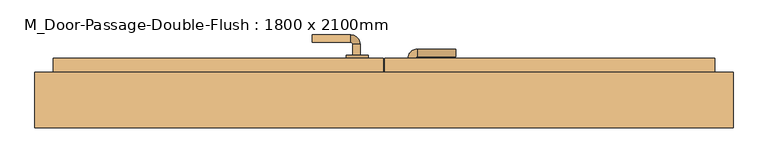
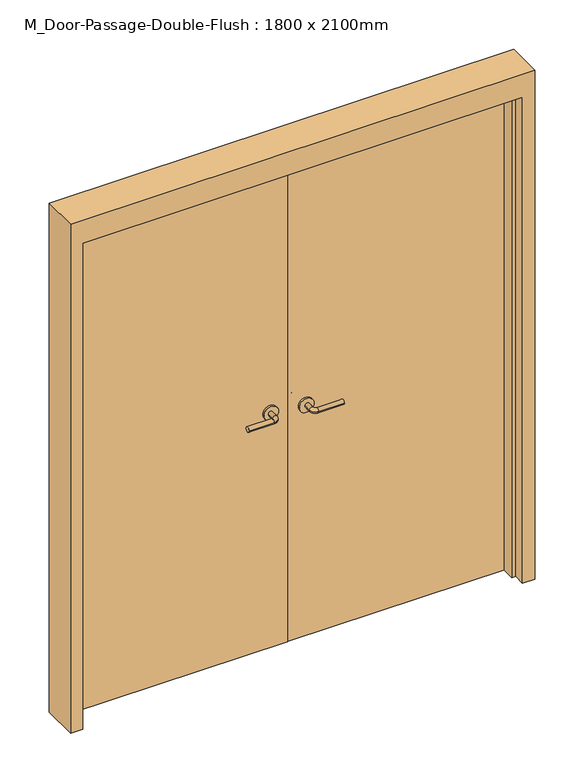
"""IFC4 building model written with IfcOpenShell, lengths in millimetres: door geometry, M_Door-Passage-Double-Flush : 1800 x 2100mm."""

from ifc_helpers import new_model, si_unit, point, frame, frame_2d, origin, origin_with_axes, place, context, project, spatial, polyline, circle_curve, ellipse_curve, trimmed, segment, composite_curve, outline, extrude, faceted_brep, source, transform, mapped, element, save
from ifc_brep_helpers import plane_surface, cylinder_surface, revolved_surface, advanced_brep


def m_door_passage_double_flush_1800_x_2100mm_c8e1a3e4(model_context):
    return source(origin(), model_context, "Body", "SolidModel", [
        advanced_brep(
        [(-65.009375, -9.15, 1016.0), (-85.009375, -9.15, 1016.0), (-65.009375, -39.15, 1016.0), (-85.009375, -39.15, 1016.0), (-90.009375, -44.15, 1016.0), (-90.009375, -64.15, 1016.0), (-195.009375, -64.15, 1016.0), (-195.009375, -44.15, 1016.0)],
        [
            (0, 1, circle_curve(frame((-75.009375, -9.15, 1016.0), z_axis=(0.0, 1.0, 0.0), x_axis=(-1.0, 0.0, 0.0)), 10.0)),
            (1, 0, circle_curve(frame((-75.009375, -9.15, 1016.0), z_axis=(0.0, 1.0, 0.0), x_axis=(-1.0, 0.0, 0.0)), 10.0)),
            (0, 2),
            (2, 3, circle_curve(frame((-75.009375, -39.15, 1016.0), z_axis=(0.0, 1.0, 0.0), x_axis=(-1.0, 0.0, 0.0)), 10.0)),
            (3, 1),
            (3, 2, circle_curve(frame((-75.009375, -39.15, 1016.0), z_axis=(0.0, 1.0, 0.0), x_axis=(-1.0, 0.0, 0.0)), 10.0)),
            (4, 3, circle_curve(frame((-90.009375, -39.15, 1016.0), z_axis=(0.0, 0.0, 1.0), x_axis=(1.0, 0.0, 0.0)), 5.0)),
            (2, 5, circle_curve(frame((-90.009375, -39.15, 1016.0), z_axis=(0.0, 0.0, -1.0), x_axis=(1.0, 0.0, 0.0)), 25.0)),
            (5, 4, circle_curve(frame((-90.009375, -54.15, 1016.0), z_axis=(1.0, 0.0, 0.0), x_axis=(0.0, 1.0, 0.0)), 10.0)),
            (4, 5, circle_curve(frame((-90.009375, -54.15, 1016.0), z_axis=(1.0, 0.0, 0.0), x_axis=(0.0, 1.0, 0.0)), 10.0)),
            (6, 7, circle_curve(frame((-195.009375, -54.15, 1016.0), z_axis=(-1.0, 0.0, 0.0), x_axis=(0.0, 1.0, 0.0)), 10.0)),
            (7, 6, circle_curve(frame((-195.009375, -54.15, 1016.0), z_axis=(-1.0, 0.0, 0.0), x_axis=(0.0, 1.0, 0.0)), 10.0)),
            (5, 6),
            (7, 4),
        ],
        [
            plane_surface(frame((-75.009375, -9.15, 1016.0), z_axis=(0.0, 1.0, 0.0), x_axis=(0.0, 0.0, 1.0))),
            cylinder_surface(frame((-75.009375, -9.15, 1016.0), z_axis=(0.0, 1.0, 0.0), x_axis=(-1.0, 0.0, 0.0)), 10.0),
            revolved_surface(trimmed(ellipse_curve(frame((-75.009375, -39.15, 1016.0), z_axis=(0.0, 1.0, 0.0), x_axis=(-1.0, 0.0, 0.0)), 10.0, 10.0), [point((-65.009375, -39.15, 1016.0))], [point((-85.009375, -39.15, 1016.0))], True, "CARTESIAN"), (-90.009375, -39.15, 1016.0), (0.0, 0.0, -1.0)),
            revolved_surface(trimmed(ellipse_curve(frame((-75.009375, -39.15, 1016.0), z_axis=(0.0, 1.0, 0.0), x_axis=(-1.0, 0.0, 0.0)), 10.0, 10.0), [point((-85.009375, -39.15, 1016.0))], [point((-65.009375, -39.15, 1016.0))], True, "CARTESIAN"), (-90.009375, -39.15, 1016.0), (0.0, 0.0, -1.0)),
            plane_surface(frame((-195.009375, -54.15, 1016.0), z_axis=(-1.0, 0.0, 0.0), x_axis=(0.0, 0.0, 1.0))),
            cylinder_surface(frame((-90.009375, -54.15, 1016.0), z_axis=(1.0, 0.0, 0.0), x_axis=(0.0, 1.0, 0.0)), 10.0),
        ],
        [
            (0, [[1, 2]]),
            (1, [[-1, 3, 4, 5]]),
            (1, [[-2, -5, 6, -3]]),
            (2, [[7, -4, 8, 9]]),
            (3, [[-8, -6, -7, 10]]),
            (4, [[11, 12]]),
            (5, [[-9, 13, -12, 14]]),
            (5, [[-10, -14, -11, -13]]),
        ],
    ),
        extrude(outline(composite_curve([segment(trimmed(circle_curve(frame_2d((1016.0, -72.509375)), 30.0), [point((1016.0, -42.509375))], [point((1016.0, -102.509375))], False, "CARTESIAN"), True, "CONTINUOUS"), segment(trimmed(circle_curve(frame_2d((1016.0, -72.509375)), 30.0), [point((1016.0, -102.509375))], [point((1016.0, -42.509375))], False, "CARTESIAN"), True, "CONTINUOUS")], self_intersect=False)), frame((0.0, -9.15, 0.0), z_axis=(0.0, 1.0, 0.0), x_axis=(0.0, 0.0, 1.0)), (0.0, 0.0, 1.0), 8.0),
        advanced_brep(
        [(-65.009375, 90.95, 1000.0), (-85.009375, 90.95, 1000.0), (-85.009375, 120.95, 1000.0), (-65.009375, 120.95, 1000.0), (-90.009375, 125.95, 1000.0), (-90.009375, 145.95, 1000.0), (-195.009375, 145.95, 1000.0), (-195.009375, 125.95, 1000.0)],
        [
            (0, 1, circle_curve(frame((-75.009375, 90.95, 1000.0), z_axis=(0.0, -1.0, 0.0), x_axis=(-1.0, 0.0, 0.0)), 10.0)),
            (1, 0, circle_curve(frame((-75.009375, 90.95, 1000.0), z_axis=(0.0, -1.0, 0.0), x_axis=(-1.0, 0.0, 0.0)), 10.0)),
            (1, 2),
            (2, 3, circle_curve(frame((-75.009375, 120.95, 1000.0), z_axis=(0.0, -1.0, 0.0), x_axis=(-1.0, 0.0, 0.0)), 10.0)),
            (3, 0),
            (3, 2, circle_curve(frame((-75.009375, 120.95, 1000.0), z_axis=(0.0, -1.0, 0.0), x_axis=(-1.0, 0.0, 0.0)), 10.0)),
            (4, 5, circle_curve(frame((-90.009375, 135.95, 1000.0), z_axis=(1.0, 0.0, 0.0), x_axis=(0.0, -1.0, 0.0)), 10.0)),
            (5, 3, circle_curve(frame((-90.009375, 120.95, 1000.0), z_axis=(0.0, 0.0, -1.0), x_axis=(1.0, 0.0, 0.0)), 25.0)),
            (2, 4, circle_curve(frame((-90.009375, 120.95, 1000.0), z_axis=(0.0, 0.0, 1.0), x_axis=(1.0, 0.0, 0.0)), 5.0)),
            (5, 4, circle_curve(frame((-90.009375, 135.95, 1000.0), z_axis=(1.0, 0.0, 0.0), x_axis=(0.0, -1.0, 0.0)), 10.0)),
            (6, 7, circle_curve(frame((-195.009375, 135.95, 1000.0), z_axis=(-1.0, 0.0, 0.0), x_axis=(0.0, -1.0, 0.0)), 10.0)),
            (7, 6, circle_curve(frame((-195.009375, 135.95, 1000.0), z_axis=(-1.0, 0.0, 0.0), x_axis=(0.0, -1.0, 0.0)), 10.0)),
            (4, 7),
            (6, 5),
        ],
        [
            plane_surface(frame((-75.009375, 90.95, 1000.0), z_axis=(0.0, -1.0, 0.0), x_axis=(0.0, 0.0, 1.0))),
            cylinder_surface(frame((-75.009375, 90.95, 1000.0), z_axis=(0.0, -1.0, 0.0), x_axis=(-1.0, 0.0, 0.0)), 10.0),
            revolved_surface(trimmed(ellipse_curve(frame((-75.009375, 120.95, 1000.0), z_axis=(0.0, 1.0, 0.0), x_axis=(-1.0, 0.0, 0.0)), 10.0, 10.0), [point((-65.009375, 120.95, 1000.0))], [point((-85.009375, 120.95, 1000.0))], True, "CARTESIAN"), (-90.009375, 120.95, 1000.0), (0.0, 0.0, -1.0)),
            revolved_surface(trimmed(ellipse_curve(frame((-75.009375, 120.95, 1000.0), z_axis=(0.0, 1.0, 0.0), x_axis=(-1.0, 0.0, 0.0)), 10.0, 10.0), [point((-85.009375, 120.95, 1000.0))], [point((-65.009375, 120.95, 1000.0))], True, "CARTESIAN"), (-90.009375, 120.95, 1000.0), (0.0, 0.0, -1.0)),
            plane_surface(frame((-195.009375, 135.95, 1000.0), z_axis=(-1.0, 0.0, 0.0), x_axis=(0.0, 0.0, 1.0))),
            cylinder_surface(frame((-90.009375, 135.95, 1000.0), z_axis=(1.0, 0.0, 0.0), x_axis=(0.0, -1.0, 0.0)), 10.0),
        ],
        [
            (0, [[1, 2]]),
            (1, [[3, 4, 5, -2]]),
            (1, [[-5, 6, -3, -1]]),
            (2, [[7, 8, -4, 9]]),
            (3, [[10, -9, -6, -8]]),
            (4, [[11, 12]]),
            (5, [[13, -11, 14, -7]]),
            (5, [[-14, -12, -13, -10]]),
        ],
    ),
        extrude(outline(composite_curve([segment(trimmed(circle_curve(frame_2d((1000.0, -72.509375)), 30.0), [point((1000.0, -42.509375))], [point((1000.0, -102.509375))], False, "CARTESIAN"), True, "CONTINUOUS"), segment(trimmed(circle_curve(frame_2d((1000.0, -72.509375)), 30.0), [point((1000.0, -102.509375))], [point((1000.0, -42.509375))], False, "CARTESIAN"), True, "CONTINUOUS")], self_intersect=False)), frame((0.0, 82.95, 0.0), z_axis=(0.0, 1.0, 0.0), x_axis=(0.0, 0.0, 1.0)), (0.0, 0.0, 1.0), 8.0),
        advanced_brep(
        [(65.009375, -9.15, 1000.0), (85.009375, -9.15, 1000.0), (85.009375, -39.15, 1000.0), (65.009375, -39.15, 1000.0), (90.009375, -44.15, 1000.0), (90.009375, -64.15, 1000.0), (195.009375, -64.15, 1000.0), (195.009375, -44.15, 1000.0)],
        [
            (0, 1, circle_curve(frame((75.009375, -9.15, 1000.0), z_axis=(0.0, 1.0, 0.0), x_axis=(1.0, 0.0, 0.0)), 10.0)),
            (1, 0, circle_curve(frame((75.009375, -9.15, 1000.0), z_axis=(0.0, 1.0, 0.0), x_axis=(1.0, 0.0, 0.0)), 10.0)),
            (1, 2),
            (2, 3, circle_curve(frame((75.009375, -39.15, 1000.0), z_axis=(0.0, 1.0, 0.0), x_axis=(1.0, 0.0, 0.0)), 10.0)),
            (3, 0),
            (3, 2, circle_curve(frame((75.009375, -39.15, 1000.0), z_axis=(0.0, 1.0, 0.0), x_axis=(1.0, 0.0, 0.0)), 10.0)),
            (4, 5, circle_curve(frame((90.009375, -54.15, 1000.0), z_axis=(-1.0, 0.0, 0.0), x_axis=(0.0, 1.0, 0.0)), 10.0)),
            (5, 3, circle_curve(frame((90.009375, -39.15, 1000.0), z_axis=(0.0, 0.0, -1.0), x_axis=(-1.0, 0.0, 0.0)), 25.0)),
            (2, 4, circle_curve(frame((90.009375, -39.15, 1000.0), z_axis=(0.0, 0.0, 1.0), x_axis=(-1.0, 0.0, 0.0)), 5.0)),
            (5, 4, circle_curve(frame((90.009375, -54.15, 1000.0), z_axis=(-1.0, 0.0, 0.0), x_axis=(0.0, 1.0, 0.0)), 10.0)),
            (6, 7, circle_curve(frame((195.009375, -54.15, 1000.0), z_axis=(1.0, 0.0, 0.0), x_axis=(0.0, 1.0, 0.0)), 10.0)),
            (7, 6, circle_curve(frame((195.009375, -54.15, 1000.0), z_axis=(1.0, 0.0, 0.0), x_axis=(0.0, 1.0, 0.0)), 10.0)),
            (4, 7),
            (6, 5),
        ],
        [
            plane_surface(frame((75.009375, -9.15, 1000.0), z_axis=(0.0, 1.0, 0.0), x_axis=(0.0, 0.0, 1.0))),
            cylinder_surface(frame((75.009375, -9.15, 1000.0), z_axis=(0.0, 1.0, 0.0), x_axis=(1.0, 0.0, 0.0)), 10.0),
            revolved_surface(trimmed(ellipse_curve(frame((75.009375, -39.15, 1000.0), z_axis=(0.0, -1.0, 0.0), x_axis=(1.0, 0.0, 0.0)), 10.0, 10.0), [point((65.009375, -39.15, 1000.0))], [point((85.009375, -39.15, 1000.0))], True, "CARTESIAN"), (90.009375, -39.15, 1000.0), (0.0, 0.0, -1.0)),
            revolved_surface(trimmed(ellipse_curve(frame((75.009375, -39.15, 1000.0), z_axis=(0.0, -1.0, 0.0), x_axis=(1.0, 0.0, 0.0)), 10.0, 10.0), [point((85.009375, -39.15, 1000.0))], [point((65.009375, -39.15, 1000.0))], True, "CARTESIAN"), (90.009375, -39.15, 1000.0), (0.0, 0.0, -1.0)),
            plane_surface(frame((195.009375, -54.15, 1000.0), z_axis=(1.0, 0.0, 0.0), x_axis=(0.0, 0.0, 1.0))),
            cylinder_surface(frame((90.009375, -54.15, 1000.0), z_axis=(-1.0, 0.0, 0.0), x_axis=(0.0, 1.0, 0.0)), 10.0),
        ],
        [
            (0, [[1, 2]]),
            (1, [[3, 4, 5, -2]]),
            (1, [[-5, 6, -3, -1]]),
            (2, [[7, 8, -4, 9]]),
            (3, [[10, -9, -6, -8]]),
            (4, [[11, 12]]),
            (5, [[13, -11, 14, -7]]),
            (5, [[-14, -12, -13, -10]]),
        ],
    ),
        extrude(outline(composite_curve([segment(trimmed(circle_curve(frame_2d((1000.0, 72.509375)), 30.0), [point((1000.0, 42.509375))], [point((1000.0, 102.509375))], False, "CARTESIAN"), True, "CONTINUOUS"), segment(trimmed(circle_curve(frame_2d((1000.0, 72.509375)), 30.0), [point((1000.0, 102.509375))], [point((1000.0, 42.509375))], False, "CARTESIAN"), True, "CONTINUOUS")], self_intersect=False)), frame((0.0, -9.15, 0.0), z_axis=(0.0, 1.0, 0.0), x_axis=(0.0, 0.0, 1.0)), (0.0, 0.0, 1.0), 8.0),
        advanced_brep(
        [(65.009375, 51.85, 1000.0), (85.009375, 51.85, 1000.0), (65.009375, 81.85, 1000.0), (85.009375, 81.85, 1000.0), (90.009375, 86.85, 1000.0), (90.009375, 106.85, 1000.0), (195.009375, 106.85, 1000.0), (195.009375, 86.85, 1000.0)],
        [
            (0, 1, circle_curve(frame((75.009375, 51.85, 1000.0), z_axis=(0.0, -1.0, 0.0), x_axis=(1.0, 0.0, 0.0)), 10.0)),
            (1, 0, circle_curve(frame((75.009375, 51.85, 1000.0), z_axis=(0.0, -1.0, 0.0), x_axis=(1.0, 0.0, 0.0)), 10.0)),
            (0, 2),
            (2, 3, circle_curve(frame((75.009375, 81.85, 1000.0), z_axis=(0.0, -1.0, 0.0), x_axis=(1.0, 0.0, 0.0)), 10.0)),
            (3, 1),
            (3, 2, circle_curve(frame((75.009375, 81.85, 1000.0), z_axis=(0.0, -1.0, 0.0), x_axis=(1.0, 0.0, 0.0)), 10.0)),
            (4, 3, circle_curve(frame((90.009375, 81.85, 1000.0), z_axis=(0.0, 0.0, 1.0), x_axis=(-1.0, 0.0, 0.0)), 5.0)),
            (2, 5, circle_curve(frame((90.009375, 81.85, 1000.0), z_axis=(0.0, 0.0, -1.0), x_axis=(-1.0, 0.0, 0.0)), 25.0)),
            (5, 4, circle_curve(frame((90.009375, 96.85, 1000.0), z_axis=(-1.0, 0.0, 0.0), x_axis=(0.0, -1.0, 0.0)), 10.0)),
            (4, 5, circle_curve(frame((90.009375, 96.85, 1000.0), z_axis=(-1.0, 0.0, 0.0), x_axis=(0.0, -1.0, 0.0)), 10.0)),
            (6, 7, circle_curve(frame((195.009375, 96.85, 1000.0), z_axis=(1.0, 0.0, 0.0), x_axis=(0.0, -1.0, 0.0)), 10.0)),
            (7, 6, circle_curve(frame((195.009375, 96.85, 1000.0), z_axis=(1.0, 0.0, 0.0), x_axis=(0.0, -1.0, 0.0)), 10.0)),
            (5, 6),
            (7, 4),
        ],
        [
            plane_surface(frame((75.009375, 51.85, 1000.0), z_axis=(0.0, -1.0, 0.0), x_axis=(0.0, 0.0, 1.0))),
            cylinder_surface(frame((75.009375, 51.85, 1000.0), z_axis=(0.0, -1.0, 0.0), x_axis=(1.0, 0.0, 0.0)), 10.0),
            revolved_surface(trimmed(ellipse_curve(frame((75.009375, 81.85, 1000.0), z_axis=(0.0, -1.0, 0.0), x_axis=(1.0, 0.0, 0.0)), 10.0, 10.0), [point((65.009375, 81.85, 1000.0))], [point((85.009375, 81.85, 1000.0))], True, "CARTESIAN"), (90.009375, 81.85, 1000.0), (0.0, 0.0, -1.0)),
            revolved_surface(trimmed(ellipse_curve(frame((75.009375, 81.85, 1000.0), z_axis=(0.0, -1.0, 0.0), x_axis=(1.0, 0.0, 0.0)), 10.0, 10.0), [point((85.009375, 81.85, 1000.0))], [point((65.009375, 81.85, 1000.0))], True, "CARTESIAN"), (90.009375, 81.85, 1000.0), (0.0, 0.0, -1.0)),
            plane_surface(frame((195.009375, 96.85, 1000.0), z_axis=(1.0, 0.0, 0.0), x_axis=(0.0, 0.0, 1.0))),
            cylinder_surface(frame((90.009375, 96.85, 1000.0), z_axis=(-1.0, 0.0, 0.0), x_axis=(0.0, -1.0, 0.0)), 10.0),
        ],
        [
            (0, [[1, 2]]),
            (1, [[-1, 3, 4, 5]]),
            (1, [[-2, -5, 6, -3]]),
            (2, [[7, -4, 8, 9]]),
            (3, [[-8, -6, -7, 10]]),
            (4, [[11, 12]]),
            (5, [[-9, 13, -12, 14]]),
            (5, [[-10, -14, -11, -13]]),
        ],
    ),
        extrude(outline(composite_curve([segment(trimmed(circle_curve(frame_2d((1000.0, 72.509375)), 30.0), [point((1000.0, 42.509375))], [point((1000.0, 102.509375))], False, "CARTESIAN"), True, "CONTINUOUS"), segment(trimmed(circle_curve(frame_2d((1000.0, 72.509375)), 30.0), [point((1000.0, 102.509375))], [point((1000.0, 42.509375))], False, "CARTESIAN"), True, "CONTINUOUS")], self_intersect=False)), frame((0.0, 43.85, 0.0), z_axis=(0.0, 1.0, 0.0), x_axis=(0.0, 0.0, 1.0)), (0.0, 0.0, 1.0), 8.0),
        extrude(outline(polyline([(900.0, -1.15), (1.5875, -1.15), (1.5875, 82.95), (900.0, 82.95), (900.0, -1.15)])), origin_with_axes(), (0.0, 0.0, 1.0), 2100.0),
        extrude(outline(polyline([(-1.5875, -1.15), (-900.0, -1.15), (-900.0, 82.95), (-1.5875, 82.95), (-1.5875, -1.15)])), origin_with_axes(), (0.0, 0.0, 1.0), 2100.0),
        faceted_brep([(900.0, -5.9125, 0.0), (900.0, 43.85, 0.0), (950.0, 43.85, 0.0), (950.0, -106.15, 0.0), (900.0, -106.15, 0.0), (900.0, -56.9375, 0.0), (884.125, -56.9375, 0.0), (884.125, -5.9125, 0.0), (900.0, -5.9125, 2100.0), (900.0, 43.85, 2100.0), (-900.0, 43.85, 2100.0), (-900.0, 43.85, 0.0), (-950.0, 43.85, 0.0), (-950.0, 43.85, 2200.0), (950.0, 43.85, 2200.0), (950.0, -106.15, 2200.0), (-950.0, -106.15, 2200.0), (-950.0, -106.15, 0.0), (-900.0, -106.15, 0.0), (-900.0, -106.15, 2100.0), (900.0, -106.15, 2100.0), (900.0, -56.9375, 2100.0), (-900.0, -56.9375, 2100.0), (-900.0, -56.9375, 0.0), (-884.125, -56.9375, 0.0), (-884.125, -56.9375, 2084.125), (884.125, -56.9375, 2084.125), (884.125, -5.9125, 2084.125), (-884.125, -5.9125, 2084.125), (-884.125, -5.9125, 0.0), (-900.0, -5.9125, 0.0), (-900.0, -5.9125, 2100.0)], [[[0, 1, 2, 3, 4, 5, 6, 7]], [[1, 0, 8, 9]], [[2, 1, 9, 10, 11, 12, 13, 14]], [[3, 2, 14, 15]], [[4, 3, 15, 16, 17, 18, 19, 20]], [[5, 4, 20, 21]], [[6, 5, 21, 22, 23, 24, 25, 26]], [[7, 6, 26, 27]], [[0, 7, 27, 28, 29, 30, 31, 8]], [[9, 8, 31, 10]], [[20, 19, 22, 21]], [[26, 25, 28, 27]], [[12, 11, 30, 29, 24, 23, 18, 17]], [[11, 10, 31, 30]], [[13, 12, 17, 16]], [[19, 18, 23, 22]], [[25, 24, 29, 28]], [[15, 14, 13, 16]]]),
    ])


if __name__ == "__main__":
    model = new_model("IFC4")
    model_context = context("Model", 3, world=origin())
    ifc_project = project(units=[si_unit("LENGTHUNIT", "METRE", prefix="MILLI")], contexts=[model_context])
    site = spatial("IfcSite", under=ifc_project)
    building = spatial("IfcBuilding", under=site)
    placement = place(None, origin())
    m_door_passage_double_flush_1800_x_2100mm_shape = m_door_passage_double_flush_1800_x_2100mm_c8e1a3e4(model_context)
    element("IfcDoor", 1, ObjectType="M_Door-Passage-Double-Flush : 1800 x 2100mm", at=placement, inside=building, context=model_context, shape_type="MappedRepresentation", body=[
        mapped(m_door_passage_double_flush_1800_x_2100mm_shape, transform((0.0, 0.0, 0.0), x_axis=(1.0, 0.0, 0.0), y_axis=(0.0, 1.0, 0.0), z_axis=(0.0, 0.0, 1.0))),
    ])
    save(model, "model.ifc")

# Revit data of these elements
# Type "M_Door-Passage-Double-Flush : 1800 x 2100mm"
#   Type Mark = "34"
#   Assembly Code = "B2030200"
#   Analytic Construction = "Metal"
#   Thickness = 45 mm
#   Thermal Resistance (R) = 0.270118 (m²·K)/W
#   Swing Angle [instance default] = 90.00°
#   Strike Height = 1000 mm
#   SinglePanelWidth = 900 mm
#   Rough Width [instance default] = 1900 mm
#   Rough Height [instance default] = 2200 mm
#   MFOpeningHeight [instance default] = 100 mm
#   MFOpeningWidth [instance default] = 100 mm
#   Inset Calculate [instance default] = 105 mm
#   Masonry Inset [instance default] = 25 mm
#   Height = 2100 mm
#   Width = 1800 mm
#   Heat Transfer Coefficient (U) = 3.70223 W/(m²·K)
#   Masonry Frame Depth = 150 mm
#   Masonry Frame [instance default] = yes
#   Function = 1
#   Dry Wall Frame [instance default] = no
#   Panel Material = Metal Door - Brindle
#   Frame Material = Metal - Painted - Grey
#   Door Handle Material = Aluminum
#   Visual Light Transmittance = 0
#   Solar Heat Gain Coefficient = 0
#   Wall Closure = (empty or 0)
# Element 1 (IfcDoor, "M_Door-Passage-Double-Flush : 1800 x 2100mm")
#   Materials on its faces: "Aluminum", "Metal - Painted - Grey", "Metal Door - Brindle"
# Materials
#   "Metal Door - Brindle": class "Paint", colour RGB 164 133 98, transparency 0
#   "Metal - Painted - Grey": class "Paint", colour RGB 104 104 104, transparency 0
#   "Aluminum": class "Metal", colour RGB 244 245 246, transparency 0, Description = "Aluminum 6061", Cost = 0
